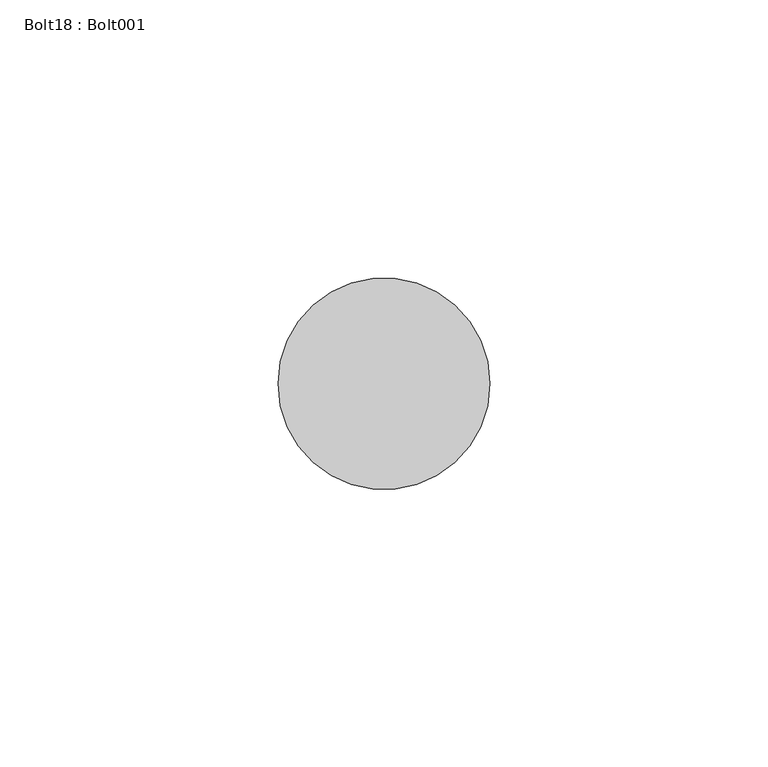
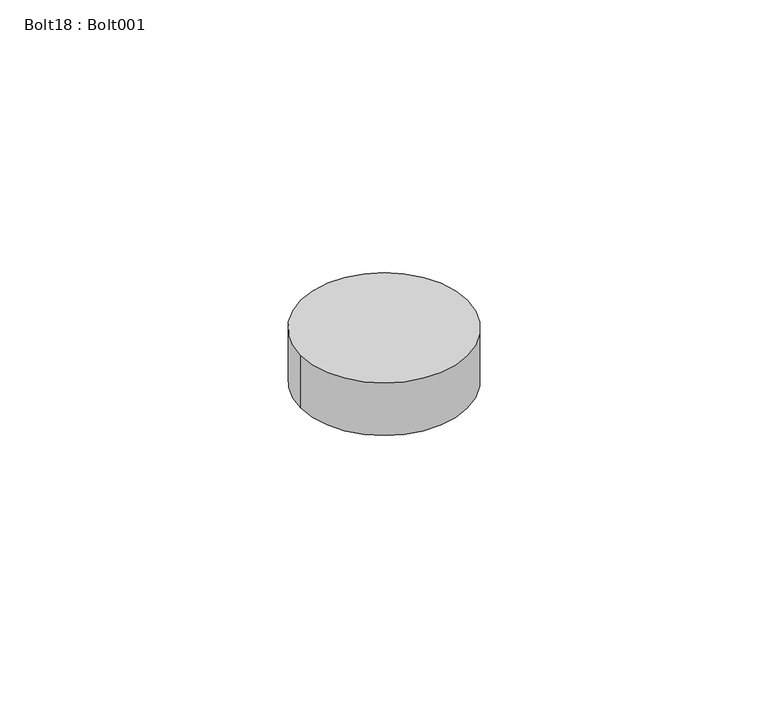
"""IFC4 building model written with IfcOpenShell, lengths in millimetres: proxy geometry, Bolt18 : Bolt001."""

from ifc_helpers import new_model, si_unit, point, frame, frame_2d, origin, place, context, project, spatial, circle_curve, trimmed, segment, composite_curve, outline, extrude, source, transform, mapped, element, save


def bolt18_bolt001_70c8ac4d(model_context):
    return source(origin(), model_context, "Body", "SweptSolid", [
        extrude(outline(composite_curve([segment(trimmed(circle_curve(frame_2d((7251.9702148, -1781.8449707)), 19.05), [point((7232.9202148, -1781.8449707))], [point((7271.0202148, -1781.8449707))], False, "CARTESIAN"), True, "CONTINUOUS"), segment(trimmed(circle_curve(frame_2d((7251.9702148, -1781.8449707)), 19.05), [point((7271.0202148, -1781.8449707))], [point((7232.9202148, -1781.8449707))], False, "CARTESIAN"), True, "CONTINUOUS")], self_intersect=False)), frame((0.0, 0.0, 40112.696), z_axis=(0.0, 0.0, 1.0), x_axis=(1.0, 0.0, 0.0)), (0.0, 0.0, 1.0), 12.7),
    ])


if __name__ == "__main__":
    model = new_model("IFC4")
    model_context = context("Model", 3, world=origin())
    ifc_project = project(units=[si_unit("LENGTHUNIT", "METRE", prefix="MILLI")], contexts=[model_context])
    site = spatial("IfcSite", under=ifc_project)
    building = spatial("IfcBuilding", under=site)
    placement = place(None, origin())
    bolt18_bolt001_shape = bolt18_bolt001_70c8ac4d(model_context)
    element("IfcBuildingElementProxy", 1, Name="Bolt18 : Bolt001", ObjectType="Bolt18 : Bolt001", at=placement, inside=building, context=model_context, shape_type="MappedRepresentation", body=[
        mapped(bolt18_bolt001_shape, transform((0.0, 0.0, 0.0), x_axis=(1.0, 0.0, 0.0), y_axis=(0.0, 1.0, 0.0), z_axis=(0.0, 0.0, 1.0))),
    ])
    save(model, "model.ifc")

# Revit data of these elements
# Type "Bolt18 : Bolt001"
#   NameOverride = "Bolt001"
# Element 1 (IfcBuildingElementProxy, "Bolt18 : Bolt001")
#   Materials on its faces: "BOLTS CONCEALED BY FLOOR FINISH"
# Materials
#   "BOLTS CONCEALED BY FLOOR FINISH": class "Unassigned", colour RGB 128 128 128, transparency 0
